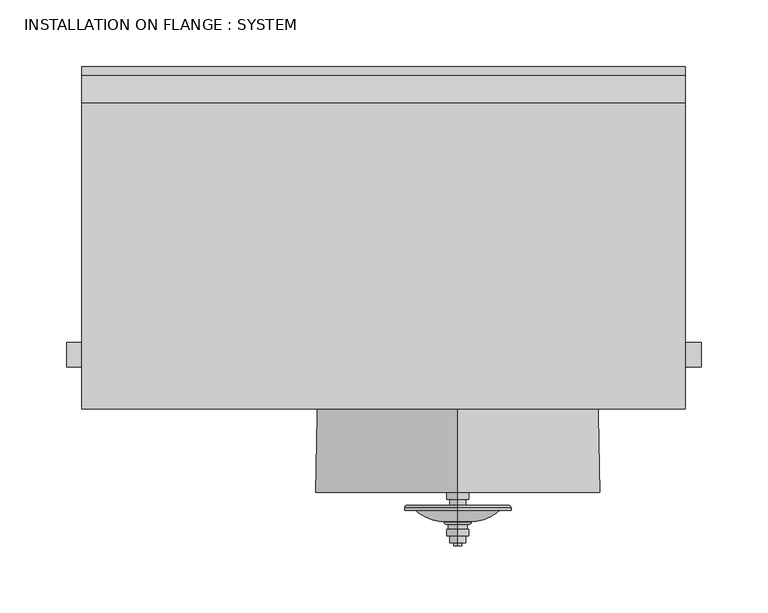
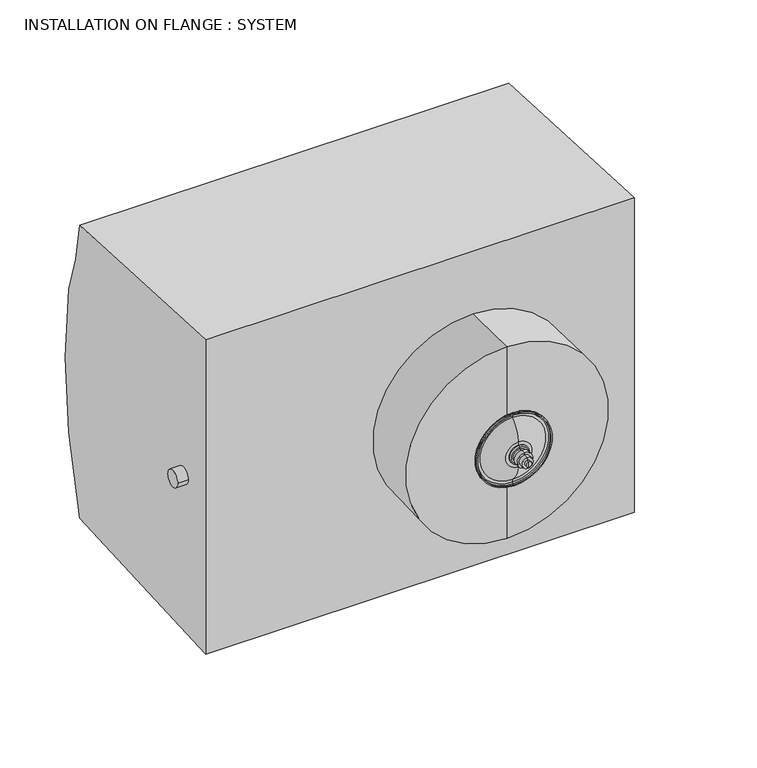
"""IFC4 building model written with IfcOpenShell, lengths in millimetres: proxy geometry, INSTALLATION ON FLANGE : SYSTEM."""

from ifc_helpers import new_model, si_unit, point, frame, frame_2d, origin, place, context, project, spatial, polyline, circle_curve, ellipse_curve, trimmed, segment, composite_curve, outline, extrude, source, transform, mapped, element, save
from ifc_brep_helpers import plane_surface, cylinder_surface, revolved_surface, spline_curve, advanced_brep


def installation_on_flange_system_eb3966a4(model_context):
    return source(origin(), model_context, "Body", "SolidModel", [
        extrude(outline(composite_curve([segment(trimmed(circle_curve(frame_2d((190.7040749, 2399.7866991)), 9.122304), [point((199.8263789, 2399.7866991))], [point((181.5817709, 2399.7866991))], False, "CARTESIAN"), True, "CONTINUOUS"), segment(trimmed(circle_curve(frame_2d((190.7040749, 2399.7866991)), 9.122304), [point((181.5817709, 2399.7866991))], [point((199.8263789, 2399.7866991))], False, "CARTESIAN"), True, "CONTINUOUS")], self_intersect=False)), frame((-167.6421762, 0.0, 0.0), z_axis=(1.0, 0.0, 0.0), x_axis=(0.0, 1.0, 0.0)), (0.0, 0.0, 1.0), 11.0317707),
        extrude(outline(composite_curve([segment(trimmed(circle_curve(frame_2d((190.7040749, 2399.7866991)), 9.122304), [point((199.8263789, 2399.7866991))], [point((181.5817709, 2399.7866991))], False, "CARTESIAN"), True, "CONTINUOUS"), segment(trimmed(circle_curve(frame_2d((190.7040749, 2399.7866991)), 9.122304), [point((181.5817709, 2399.7866991))], [point((199.8263789, 2399.7866991))], False, "CARTESIAN"), True, "CONTINUOUS")], self_intersect=False)), frame((295.4714703, 0.0, 0.0), z_axis=(1.0, 0.0, 0.0), x_axis=(0.0, 1.0, 0.0)), (0.0, 0.0, 1.0), 11.8217179),
        extrude(outline(composite_curve([segment(polyline([(379.684793, 2236.9784241), (150.0, 2224.9411541), (150.0, 2574.9411541), (379.684793, 2563.5501198)]), True, "CONTINUOUS"), segment(trimmed(circle_curve(frame_2d((720.4699006, 2602.8642327)), 343.0453163), [point((379.684793, 2563.5501198))], [point((400.2189468, 2479.9031999))], True, "CARTESIAN"), True, "CONTINUOUS"), segment(trimmed(circle_curve(frame_2d((-104.831346, 2400.2642719)), 511.2906777), [point((400.2189468, 2479.9031999))], [point((400.1449827, 2320.15769))], False, "CARTESIAN"), True, "CONTINUOUS"), segment(trimmed(circle_curve(frame_2d((874.3507266, 2159.4079627)), 500.7110568), [point((400.1449827, 2320.15769))], [point((379.684793, 2236.9784241))], True, "CARTESIAN"), True, "CONTINUOUS")], self_intersect=False)), frame((-156.6104055, 0.0, 0.0), z_axis=(1.0, 0.0, 0.0), x_axis=(0.0, 1.0, 0.0)), (0.0, 0.0, 1.0), 452.0818758),
        advanced_brep(
        [(125.0, 49.800001, 2396.9974459), (125.0, 49.800001, 2403.0025541), (125.0, 47.5000006, 2403.0025541), (125.0, 47.5000006, 2396.9974459), (125.0, 49.800001, 2394.1058972), (125.0, 49.800001, 2405.8941028), (125.0, 54.9999993, 2394.1058972), (125.0, 54.9999993, 2405.8941028), (125.0, 54.9999993, 2391.7764643), (125.0, 54.9999993, 2408.2235357), (125.0, 60.0000007, 2391.7764643), (125.0, 60.0000007, 2408.2235357), (125.0, 60.0000007, 2392.7564219), (125.0, 60.0000007, 2407.2435781), (125.0, 63.8000004, 2392.7564219), (125.0, 63.8000004, 2407.2435781), (125.0, 63.8000004, 2391.0662237), (125.0, 63.8000004, 2408.9337763), (125.0, 65.1302816, 2389.7691944), (125.0, 65.1302816, 2410.2308056), (125.0, 65.9854344, 2389.7691944), (125.0, 65.9854344, 2410.2308056), (125.0, 65.9854344, 2386.2784266), (125.0, 65.9854344, 2413.7215734), (125.0, 76.7999995, 2365.472179), (125.0, 76.7999995, 2434.527821), (125.0, 76.7999995, 2362.519154), (125.0, 76.7999995, 2437.480846), (125.0, 75.9940284, 2361.2128962), (125.0, 75.9940284, 2438.7871038), (125.0, 74.0999996, 2361.2128962), (125.0, 74.0999996, 2438.7871038), (125.0, 74.0999996, 2360.0392013), (125.0, 74.0999996, 2439.9607987), (125.0, 75.9940284, 2360.0392013), (125.0, 75.9940284, 2439.9607987), (125.0, 78.0, 2362.0451729), (125.0, 78.0, 2437.9548271), (125.0, 78.0, 2394.1058972), (125.0, 78.0, 2405.8941028), (125.0, 82.5000002, 2394.1058972), (125.0, 82.5000002, 2405.8941028), (125.0, 82.5000002, 2391.7764643), (125.0, 82.5000002, 2408.2235357), (125.0, 87.4999999, 2391.7764643), (125.0, 87.4999999, 2408.2235357), (125.0, 87.4999999, 2293.250711), (125.0, 87.4999999, 2506.749289), (125.0, 163.9945916, 2294.5859291), (125.0, 163.9945916, 2505.4140709), (125.0, 163.9945916, 2334.5859291), (125.0, 163.9945916, 2465.4140709), (125.0, 166.1335115, 2336.724849), (125.0, 166.1335115, 2463.275151), (125.0, 166.1335115, 2400.0), (125.0, 47.5000006, 2400.0)],
        [
            (0, 1, circle_curve(frame((125.0, 49.800001, 2400.0), z_axis=(0.0, -1.0, 0.0), x_axis=(0.0, 0.0, 1.0)), 3.0025541)),
            (1, 2),
            (2, 3, circle_curve(frame((125.0, 47.5000006, 2400.0), z_axis=(0.0, 1.0, 0.0), x_axis=(0.0, 0.0, 1.0)), 3.0025541)),
            (3, 0),
            (1, 0, circle_curve(frame((125.0, 49.800001, 2400.0), z_axis=(0.0, -1.0, 0.0), x_axis=(0.0, 0.0, 1.0)), 3.0025541)),
            (3, 2, circle_curve(frame((125.0, 47.5000006, 2400.0), z_axis=(0.0, 1.0, 0.0), x_axis=(0.0, 0.0, 1.0)), 3.0025541)),
            (4, 5, circle_curve(frame((125.0, 49.800001, 2400.0), z_axis=(0.0, -1.0, 0.0), x_axis=(0.0, 0.0, 1.0)), 5.8941028)),
            (5, 1),
            (0, 4),
            (5, 4, circle_curve(frame((125.0, 49.800001, 2400.0), z_axis=(0.0, -1.0, 0.0), x_axis=(0.0, 0.0, 1.0)), 5.8941028)),
            (6, 7, circle_curve(frame((125.0, 54.9999993, 2400.0), z_axis=(0.0, -1.0, 0.0), x_axis=(0.0, 0.0, 1.0)), 5.8941028)),
            (7, 5),
            (4, 6),
            (7, 6, circle_curve(frame((125.0, 54.9999993, 2400.0), z_axis=(0.0, -1.0, 0.0), x_axis=(0.0, 0.0, 1.0)), 5.8941028)),
            (8, 9, circle_curve(frame((125.0, 54.9999993, 2400.0), z_axis=(0.0, -1.0, 0.0), x_axis=(0.0, 0.0, 1.0)), 8.2235357)),
            (9, 7),
            (6, 8),
            (9, 8, circle_curve(frame((125.0, 54.9999993, 2400.0), z_axis=(0.0, -1.0, 0.0), x_axis=(0.0, 0.0, 1.0)), 8.2235357)),
            (10, 11, circle_curve(frame((125.0, 60.0000007, 2400.0), z_axis=(0.0, -1.0, 0.0), x_axis=(0.0, 0.0, 1.0)), 8.2235357)),
            (11, 9),
            (8, 10),
            (11, 10, circle_curve(frame((125.0, 60.0000007, 2400.0), z_axis=(0.0, -1.0, 0.0), x_axis=(0.0, 0.0, 1.0)), 8.2235357)),
            (12, 13, circle_curve(frame((125.0, 60.0000007, 2400.0), z_axis=(0.0, -1.0, 0.0), x_axis=(0.0, 0.0, 1.0)), 7.2435781)),
            (13, 11),
            (10, 12),
            (13, 12, circle_curve(frame((125.0, 60.0000007, 2400.0), z_axis=(0.0, -1.0, 0.0), x_axis=(0.0, 0.0, 1.0)), 7.2435781)),
            (14, 15, circle_curve(frame((125.0, 63.8000004, 2400.0), z_axis=(0.0, -1.0, 0.0), x_axis=(0.0, 0.0, 1.0)), 7.2435781)),
            (15, 13),
            (12, 14),
            (15, 14, circle_curve(frame((125.0, 63.8000004, 2400.0), z_axis=(0.0, -1.0, 0.0), x_axis=(0.0, 0.0, 1.0)), 7.2435781)),
            (16, 17, circle_curve(frame((125.0, 63.8000004, 2400.0), z_axis=(0.0, -1.0, 0.0), x_axis=(0.0, 0.0, 1.0)), 8.9337763)),
            (17, 15),
            (14, 16),
            (17, 16, circle_curve(frame((125.0, 63.8000004, 2400.0), z_axis=(0.0, -1.0, 0.0), x_axis=(0.0, 0.0, 1.0)), 8.9337763)),
            (18, 19, circle_curve(frame((125.0, 65.1302816, 2400.0), z_axis=(0.0, -1.0, 0.0), x_axis=(0.0, 0.0, 1.0)), 10.2308056)),
            (19, 17, spline_curve(3, [(125.0, 65.1302816, 2410.2308056), (125.0, 64.408269131, 2410.18031757), (125.0, 63.964842091, 2409.747974442), (125.0, 63.8000004, 2408.9337763)], [4, 4], [0.0, 0.003825031864308585])),
            (16, 18, spline_curve(3, [(125.0, 63.8000004, 2391.0662237), (125.0, 63.964842091, 2390.252025558), (125.0, 64.408269131, 2389.81968243), (125.0, 65.1302816, 2389.7691944)], [4, 4], [0.0, 0.003825031864308585])),
            (19, 18, circle_curve(frame((125.0, 65.1302816, 2400.0), z_axis=(0.0, -1.0, 0.0), x_axis=(0.0, 0.0, 1.0)), 10.2308056)),
            (20, 21, circle_curve(frame((125.0, 65.9854344, 2400.0), z_axis=(0.0, -1.0, 0.0), x_axis=(0.0, 0.0, 1.0)), 10.2308056)),
            (21, 19),
            (18, 20),
            (21, 20, circle_curve(frame((125.0, 65.9854344, 2400.0), z_axis=(0.0, -1.0, 0.0), x_axis=(0.0, 0.0, 1.0)), 10.2308056)),
            (22, 23, circle_curve(frame((125.0, 65.9854344, 2400.0), z_axis=(0.0, -1.0, 0.0), x_axis=(0.0, 0.0, 1.0)), 13.7215734)),
            (23, 21),
            (20, 22),
            (23, 22, circle_curve(frame((125.0, 65.9854344, 2400.0), z_axis=(0.0, -1.0, 0.0), x_axis=(0.0, 0.0, 1.0)), 13.7215734)),
            (24, 25, circle_curve(frame((125.0, 76.7999995, 2400.0), z_axis=(0.0, -1.0, 0.0), x_axis=(0.0, 0.0, 1.0)), 34.527821)),
            (25, 23, spline_curve(3, [(125.0, 76.7999995, 2434.527821), (125.0, 70.192507089, 2427.920328589), (125.0, 66.587652064, 2420.984912731), (125.0, 65.9854344, 2413.7215734)], [4, 4], [0.0, 0.04037262450680565])),
            (22, 24, spline_curve(3, [(125.0, 65.9854344, 2386.2784266), (125.0, 66.587652064, 2379.015087269), (125.0, 70.192507089, 2372.079671411), (125.0, 76.7999995, 2365.472179)], [4, 4], [0.0, 0.04037262450680565])),
            (25, 24, circle_curve(frame((125.0, 76.7999995, 2400.0), z_axis=(0.0, -1.0, 0.0), x_axis=(0.0, 0.0, 1.0)), 34.527821)),
            (26, 27, circle_curve(frame((125.0, 76.7999995, 2400.0), z_axis=(0.0, -1.0, 0.0), x_axis=(0.0, 0.0, 1.0)), 37.480846)),
            (27, 25),
            (24, 26),
            (27, 26, circle_curve(frame((125.0, 76.7999995, 2400.0), z_axis=(0.0, -1.0, 0.0), x_axis=(0.0, 0.0, 1.0)), 37.480846)),
            (28, 29, circle_curve(frame((125.0, 75.9940284, 2400.0), z_axis=(0.0, -1.0, 0.0), x_axis=(0.0, 0.0, 1.0)), 38.7871038)),
            (29, 27, circle_curve(frame((125.0, 75.7143697, 2437.7127782), z_axis=(-1.0, 0.0, 0.0), x_axis=(0.0, 0.0, -1.0)), 1.1101281)),
            (26, 28, circle_curve(frame((125.0, 75.7143697, 2362.2872218), z_axis=(-1.0, 0.0, 0.0), x_axis=(0.0, 0.0, 1.0)), 1.1101281)),
            (29, 28, circle_curve(frame((125.0, 75.9940284, 2400.0), z_axis=(0.0, -1.0, 0.0), x_axis=(0.0, 0.0, 1.0)), 38.7871038)),
            (30, 31, circle_curve(frame((125.0, 74.0999996, 2400.0), z_axis=(0.0, -1.0, 0.0), x_axis=(0.0, 0.0, 1.0)), 38.7871038)),
            (31, 29),
            (28, 30),
            (31, 30, circle_curve(frame((125.0, 74.0999996, 2400.0), z_axis=(0.0, -1.0, 0.0), x_axis=(0.0, 0.0, 1.0)), 38.7871038)),
            (32, 33, circle_curve(frame((125.0, 74.0999996, 2400.0), z_axis=(0.0, -1.0, 0.0), x_axis=(0.0, 0.0, 1.0)), 39.9607987)),
            (33, 31),
            (30, 32),
            (33, 32, circle_curve(frame((125.0, 74.0999996, 2400.0), z_axis=(0.0, -1.0, 0.0), x_axis=(0.0, 0.0, 1.0)), 39.9607987)),
            (34, 35, circle_curve(frame((125.0, 75.9940284, 2400.0), z_axis=(0.0, -1.0, 0.0), x_axis=(0.0, 0.0, 1.0)), 39.9607987)),
            (35, 33),
            (32, 34),
            (35, 34, circle_curve(frame((125.0, 75.9940284, 2400.0), z_axis=(0.0, -1.0, 0.0), x_axis=(0.0, 0.0, 1.0)), 39.9607987)),
            (36, 37, circle_curve(frame((125.0, 78.0, 2400.0), z_axis=(0.0, -1.0, 0.0), x_axis=(0.0, 0.0, 1.0)), 37.9548271)),
            (37, 35, circle_curve(frame((125.0, 75.9940284, 2437.9548271), z_axis=(1.0, 0.0, 0.0), x_axis=(0.0, 0.0, -1.0)), 2.0059716)),
            (34, 36, circle_curve(frame((125.0, 75.9940284, 2362.0451729), z_axis=(1.0, 0.0, 0.0), x_axis=(0.0, 0.0, 1.0)), 2.0059716)),
            (37, 36, circle_curve(frame((125.0, 78.0, 2400.0), z_axis=(0.0, -1.0, 0.0), x_axis=(0.0, 0.0, 1.0)), 37.9548271)),
            (38, 39, circle_curve(frame((125.0, 78.0, 2400.0), z_axis=(0.0, -1.0, 0.0), x_axis=(0.0, 0.0, 1.0)), 5.8941028)),
            (39, 37),
            (36, 38),
            (39, 38, circle_curve(frame((125.0, 78.0, 2400.0), z_axis=(0.0, -1.0, 0.0), x_axis=(0.0, 0.0, 1.0)), 5.8941028)),
            (40, 41, circle_curve(frame((125.0, 82.5000002, 2400.0), z_axis=(0.0, -1.0, 0.0), x_axis=(0.0, 0.0, 1.0)), 5.8941028)),
            (41, 39),
            (38, 40),
            (41, 40, circle_curve(frame((125.0, 82.5000002, 2400.0), z_axis=(0.0, -1.0, 0.0), x_axis=(0.0, 0.0, 1.0)), 5.8941028)),
            (42, 43, circle_curve(frame((125.0, 82.5000002, 2400.0), z_axis=(0.0, -1.0, 0.0), x_axis=(0.0, 0.0, 1.0)), 8.2235357)),
            (43, 41),
            (40, 42),
            (43, 42, circle_curve(frame((125.0, 82.5000002, 2400.0), z_axis=(0.0, -1.0, 0.0), x_axis=(0.0, 0.0, 1.0)), 8.2235357)),
            (44, 45, circle_curve(frame((125.0, 87.4999999, 2400.0), z_axis=(0.0, -1.0, 0.0), x_axis=(0.0, 0.0, 1.0)), 8.2235357)),
            (45, 43),
            (42, 44),
            (45, 44, circle_curve(frame((125.0, 87.4999999, 2400.0), z_axis=(0.0, -1.0, 0.0), x_axis=(0.0, 0.0, 1.0)), 8.2235357)),
            (46, 47, circle_curve(frame((125.0, 87.4999999, 2400.0), z_axis=(0.0, -1.0, 0.0), x_axis=(0.0, 0.0, 1.0)), 106.749289)),
            (47, 45),
            (44, 46),
            (47, 46, circle_curve(frame((125.0, 87.4999999, 2400.0), z_axis=(0.0, -1.0, 0.0), x_axis=(0.0, 0.0, 1.0)), 106.749289)),
            (48, 49, circle_curve(frame((125.0, 163.9945916, 2400.0), z_axis=(0.0, -1.0, 0.0), x_axis=(0.0, 0.0, 1.0)), 105.4140709)),
            (49, 47),
            (46, 48),
            (49, 48, circle_curve(frame((125.0, 163.9945916, 2400.0), z_axis=(0.0, -1.0, 0.0), x_axis=(0.0, 0.0, 1.0)), 105.4140709)),
            (50, 51, circle_curve(frame((125.0, 163.9945916, 2400.0), z_axis=(0.0, -1.0, 0.0), x_axis=(0.0, 0.0, 1.0)), 65.4140709)),
            (51, 49),
            (48, 50),
            (51, 50, circle_curve(frame((125.0, 163.9945916, 2400.0), z_axis=(0.0, -1.0, 0.0), x_axis=(0.0, 0.0, 1.0)), 65.4140709)),
            (52, 53, circle_curve(frame((125.0, 166.1335115, 2400.0), z_axis=(0.0, -1.0, 0.0), x_axis=(0.0, 0.0, 1.0)), 63.275151)),
            (53, 51),
            (50, 52),
            (53, 52, circle_curve(frame((125.0, 166.1335115, 2400.0), z_axis=(0.0, -1.0, 0.0), x_axis=(0.0, 0.0, 1.0)), 63.275151)),
            (54, 53),
            (52, 54),
            (2, 55),
            (55, 3),
        ],
        [
            cylinder_surface(frame((125.0, -15.0, 2400.0), z_axis=(0.0, 1.0, 0.0), x_axis=(0.0, 0.0, 1.0)), 3.0025541),
            plane_surface(frame((125.0, 49.800001, 2400.0), z_axis=(0.0, -1.0, 0.0), x_axis=(0.0, 0.0, 1.0))),
            cylinder_surface(frame((125.0, -15.0, 2400.0), z_axis=(0.0, 1.0, 0.0), x_axis=(0.0, 0.0, 1.0)), 5.8941028),
            plane_surface(frame((125.0, 54.9999993, 2400.0), z_axis=(0.0, -1.0, 0.0), x_axis=(0.0, 0.0, 1.0))),
            cylinder_surface(frame((125.0, -15.0, 2400.0), z_axis=(0.0, 1.0, 0.0), x_axis=(0.0, 0.0, 1.0)), 8.2235357),
            plane_surface(frame((125.0, 60.0000007, 2400.0), z_axis=(0.0, 1.0, 0.0), x_axis=(0.0, 0.0, 1.0))),
            cylinder_surface(frame((125.0, -15.0, 2400.0), z_axis=(0.0, 1.0, 0.0), x_axis=(0.0, 0.0, 1.0)), 7.2435781),
            plane_surface(frame((125.0, 63.8000004, 2400.0), z_axis=(0.0, -1.0, 0.0), x_axis=(0.0, 0.0, 1.0))),
            revolved_surface(spline_curve(3, [(125.0, 63.8000004, 2408.9337763), (125.0, 63.964842091, 2409.747974442), (125.0, 64.408269131, 2410.18031757), (125.0, 65.1302816, 2410.2308056)], [4, 4], [0.0, 0.003825031864308585]), (125.0, -15.0, 2400.0), (0.0, 1.0, 0.0)),
            cylinder_surface(frame((125.0, -15.0, 2400.0), z_axis=(0.0, 1.0, 0.0), x_axis=(0.0, 0.0, 1.0)), 10.2308056),
            plane_surface(frame((125.0, 65.9854344, 2400.0), z_axis=(0.0, -1.0, 0.0), x_axis=(0.0, 0.0, 1.0))),
            revolved_surface(spline_curve(3, [(125.0, 65.9854344, 2413.7215734), (125.0, 66.587652064, 2420.984912731), (125.0, 70.192507089, 2427.920328589), (125.0, 76.7999995, 2434.527821)], [4, 4], [0.0, 0.04037262450680565]), (125.0, -15.0, 2400.0), (0.0, 1.0, 0.0)),
            plane_surface(frame((125.0, 76.7999995, 2400.0), z_axis=(0.0, -1.0, 0.0), x_axis=(0.0, 0.0, 1.0))),
            revolved_surface(trimmed(ellipse_curve(frame((125.0, 75.7143697, 2437.7127782), z_axis=(1.0, 0.0, 0.0), x_axis=(0.0, 0.0, -1.0)), 1.1101281, 1.1101281), [point((125.0, 76.7999995, 2437.480846))], [point((125.0, 75.9940284, 2438.7871038))], True, "CARTESIAN"), (125.0, -15.0, 2400.0), (0.0, 1.0, 0.0)),
            revolved_surface(polyline([(125.0, 75.9940284, 2438.7871038), (125.0, 74.0999996, 2438.7871038)]), (125.0, -15.0, 2400.0), (0.0, 1.0, 0.0)),
            plane_surface(frame((125.0, 74.0999996, 2400.0), z_axis=(0.0, -1.0, 0.0), x_axis=(0.0, 0.0, 1.0))),
            cylinder_surface(frame((125.0, -15.0, 2400.0), z_axis=(0.0, 1.0, 0.0), x_axis=(0.0, 0.0, 1.0)), 39.9607987),
            revolved_surface(trimmed(ellipse_curve(frame((125.0, 75.9940284, 2437.9548271), z_axis=(-1.0, 0.0, 0.0), x_axis=(0.0, 0.0, -1.0)), 2.0059716, 2.0059716), [point((125.0, 75.9940284, 2439.9607987))], [point((125.0, 78.0, 2437.9548271))], True, "CARTESIAN"), (125.0, -15.0, 2400.0), (0.0, 1.0, 0.0)),
            plane_surface(frame((125.0, 78.0, 2400.0), z_axis=(0.0, 1.0, 0.0), x_axis=(0.0, 0.0, 1.0))),
            plane_surface(frame((125.0, 82.5000002, 2400.0), z_axis=(0.0, -1.0, 0.0), x_axis=(0.0, 0.0, 1.0))),
            plane_surface(frame((125.0, 87.4999999, 2400.0), z_axis=(0.0, -1.0, 0.0), x_axis=(0.0, 0.0, 1.0))),
            revolved_surface(polyline([(125.0, 87.4999999, 2506.749289), (125.0, 163.9945916, 2505.4140709)]), (125.0, -15.0, 2400.0), (0.0, 1.0, 0.0)),
            plane_surface(frame((125.0, 163.9945916, 2400.0), z_axis=(0.0, 1.0, 0.0), x_axis=(0.0, 0.0, 1.0))),
            revolved_surface(polyline([(125.0, 163.9945916, 2465.4140709), (125.0, 166.1335115, 2463.275151)]), (125.0, -15.0, 2400.0), (0.0, 1.0, 0.0)),
            plane_surface(frame((125.0, 166.1335115, 2400.0), z_axis=(0.0, 1.0, 0.0), x_axis=(0.0, 0.0, 1.0))),
            plane_surface(frame((125.0, 47.5000006, 2400.0), z_axis=(0.0, -1.0, 0.0), x_axis=(0.0, 0.0, 1.0))),
        ],
        [
            (0, [[1, 2, 3, 4]]),
            (0, [[5, -4, 6, -2]]),
            (1, [[7, 8, -1, 9]]),
            (1, [[10, -9, -5, -8]]),
            (2, [[11, 12, -7, 13]]),
            (2, [[14, -13, -10, -12]]),
            (3, [[15, 16, -11, 17]]),
            (3, [[18, -17, -14, -16]]),
            (4, [[19, 20, -15, 21]]),
            (4, [[22, -21, -18, -20]]),
            (5, [[23, 24, -19, 25]]),
            (5, [[26, -25, -22, -24]]),
            (6, [[27, 28, -23, 29]]),
            (6, [[30, -29, -26, -28]]),
            (7, [[31, 32, -27, 33]]),
            (7, [[34, -33, -30, -32]]),
            (8, [[35, 36, -31, 37]]),
            (8, [[38, -37, -34, -36]]),
            (9, [[39, 40, -35, 41]]),
            (9, [[42, -41, -38, -40]]),
            (10, [[43, 44, -39, 45]]),
            (10, [[46, -45, -42, -44]]),
            (11, [[47, 48, -43, 49]]),
            (11, [[50, -49, -46, -48]]),
            (12, [[51, 52, -47, 53]]),
            (12, [[54, -53, -50, -52]]),
            (13, [[55, 56, -51, 57]]),
            (13, [[58, -57, -54, -56]]),
            (14, [[59, 60, -55, 61]]),
            (14, [[62, -61, -58, -60]]),
            (15, [[63, 64, -59, 65]]),
            (15, [[66, -65, -62, -64]]),
            (16, [[67, 68, -63, 69]]),
            (16, [[70, -69, -66, -68]]),
            (17, [[71, 72, -67, 73]]),
            (17, [[74, -73, -70, -72]]),
            (18, [[75, 76, -71, 77]]),
            (18, [[78, -77, -74, -76]]),
            (2, [[79, 80, -75, 81]]),
            (2, [[82, -81, -78, -80]]),
            (19, [[83, 84, -79, 85]]),
            (19, [[86, -85, -82, -84]]),
            (4, [[87, 88, -83, 89]]),
            (4, [[90, -89, -86, -88]]),
            (20, [[91, 92, -87, 93]]),
            (20, [[94, -93, -90, -92]]),
            (21, [[95, 96, -91, 97]]),
            (21, [[98, -97, -94, -96]]),
            (22, [[99, 100, -95, 101]]),
            (22, [[102, -101, -98, -100]]),
            (23, [[103, 104, -99, 105]]),
            (23, [[106, -105, -102, -104]]),
            (24, [[107, -103, 108]]),
            (24, [[-108, -106, -107]]),
            (25, [[-3, 109, 110]]),
            (25, [[-6, -110, -109]]),
        ],
    ),
    ])


if __name__ == "__main__":
    model = new_model("IFC4")
    model_context = context("Model", 3, world=origin())
    ifc_project = project(units=[si_unit("LENGTHUNIT", "METRE", prefix="MILLI")], contexts=[model_context])
    site = spatial("IfcSite", under=ifc_project)
    building = spatial("IfcBuilding", under=site)
    placement = place(None, origin())
    installation_on_flange_system_shape = installation_on_flange_system_eb3966a4(model_context)
    element("IfcBuildingElementProxy", 1, Name="INSTALLATION ON FLANGE : SYSTEM", ObjectType="INSTALLATION ON FLANGE : SYSTEM", at=placement, inside=building, context=model_context, shape_type="MappedRepresentation", body=[
        mapped(installation_on_flange_system_shape, transform((0.0, 0.0, 0.0), x_axis=(1.0, 0.0, 0.0), y_axis=(0.0, 1.0, 0.0), z_axis=(0.0, 0.0, 1.0))),
    ])
    save(model, "model.ifc")

# Revit data of these elements
# Project information
#   Project Issue Date = "Issue Date"
#   Project Status = "Project Status"
#   Client Name = "Owner"
#   Project Address = "Enter address here"
#   Project Name = "Project Name"
#   Project Number = "Project Number"
# Type "INSTALLATION ON FLANGE : SYSTEM"
#   FLANGE HEIGHT [instance default] = 2400 mm
#   SYSTEM 90* = no
#   SYSTEM = yes
#   Model = ""
#   Default Elevation = 0
